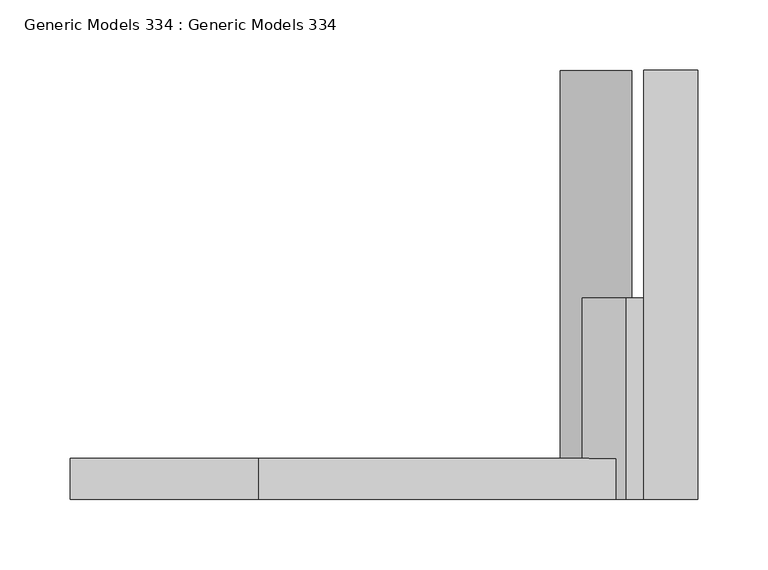
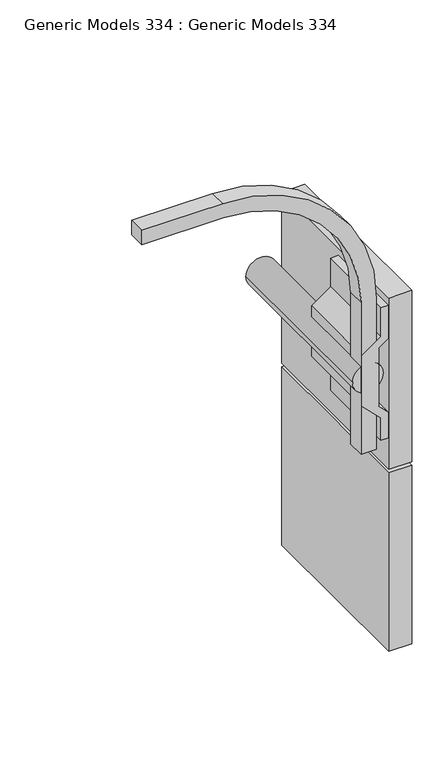
"""IFC4 building model written with IfcOpenShell, lengths in millimetres: proxy geometry, Generic Models 334 : Generic Models 334."""

from ifc_helpers import new_model, si_unit, point, frame, frame_2d, origin, place, context, project, spatial, polyline, circle_curve, trimmed, segment, composite_curve, outline, extrude, source, transform, mapped, element, save


def generic_models_334_generic_models_334_cd4350b1(model_context):
    return source(origin(), model_context, "Body", "SweptSolid", [
        extrude(outline(polyline([(126118.4886506, 8247.7371996), (126175.6386506, 8247.7371996), (126175.6386506, 8235.0371996), (126125.0998522, 8235.0371996), (126103.2465899, 8203.8275067), (126015.1748762, 8203.8275067), (125983.9651833, 8235.0371996), (125944.7756955, 8235.0371996), (125944.7756955, 8247.7371996), (125989.2256955, 8247.7371996), (126005.1885944, 8231.7743007), (126107.3113085, 8231.7743007), (126118.4886506, 8247.7371996)])), frame((0.0, -4109.6428838, 0.0), z_axis=(0.0, 1.0, 0.0), x_axis=(0.0, 0.0, 1.0)), (0.0, 0.0, 1.0), 143.0193921),
        extrude(outline(composite_curve([segment(trimmed(circle_curve(frame_2d((126060.9854905, 8213.7932071)), 25.4), [point((126060.9854905, 8239.1932071))], [point((126060.9854905, 8188.3932071))], False, "CARTESIAN"), True, "CONTINUOUS"), segment(trimmed(circle_curve(frame_2d((126060.9854905, 8213.7932071)), 25.4), [point((126060.9854905, 8188.3932071))], [point((126060.9854905, 8239.1932071))], False, "CARTESIAN"), True, "CONTINUOUS")], self_intersect=False)), frame((0.0, -4109.6428838, 0.0), z_axis=(0.0, 1.0, 0.0), x_axis=(0.0, 0.0, 1.0)), (0.0, 0.0, 1.0), 304.8),
        extrude(outline(composite_curve([segment(trimmed(circle_curve(frame_2d((126194.6886506, 7973.9169406)), 254.0), [point((126194.6886506, 8227.9169406))], [point((126448.6886506, 7973.9169406))], False, "CARTESIAN"), True, "CONTINUOUS"), segment(polyline([(126448.6886506, 7973.9169406), (126448.6886506, 7840.5669406), (126423.2886506, 7840.5669406), (126423.2886506, 7975.117678)]), True, "CONTINUOUS"), segment(trimmed(circle_curve(frame_2d((126194.6886506, 7973.9169406)), 228.6031535), [point((126423.2886506, 7975.117678))], [point((126195.8893881, 8202.5169406))], True, "CARTESIAN"), True, "CONTINUOUS"), segment(polyline([(126195.8893881, 8202.5169406), (125931.2571139, 8202.5169406), (125931.2571139, 8227.9169406), (126194.6886506, 8227.9169406)]), True, "CONTINUOUS")], self_intersect=False)), frame((0.0, -4109.6428838, 0.0), z_axis=(0.0, 1.0, 0.0), x_axis=(0.0, 0.0, 1.0)), (0.0, 0.0, 1.0), 28.9445755),
        extrude(outline(polyline([(8247.7371996, -3804.8428838), (8285.8371996, -3804.8428838), (8285.8371996, -4109.6428838), (8247.7371996, -4109.6428838), (8247.7371996, -3804.8428838)])), frame((0.0, 0.0, 125572.0903036), z_axis=(0.0, 0.0, 1.0), x_axis=(1.0, 0.0, 0.0)), (0.0, 0.0, 1.0), 311.15),
        extrude(outline(polyline([(8247.7371996, -3804.8428838), (8285.8371996, -3804.8428838), (8285.8371996, -4109.6428838), (8247.7371996, -4109.6428838), (8247.7371996, -3804.8428838)])), frame((0.0, 0.0, 125889.5903036), z_axis=(0.0, 0.0, 1.0), x_axis=(1.0, 0.0, 0.0)), (0.0, 0.0, 1.0), 298.45),
    ])


if __name__ == "__main__":
    model = new_model("IFC4")
    model_context = context("Model", 3, world=origin())
    ifc_project = project(units=[si_unit("LENGTHUNIT", "METRE", prefix="MILLI")], contexts=[model_context])
    site = spatial("IfcSite", under=ifc_project)
    building = spatial("IfcBuilding", under=site)
    placement = place(None, origin())
    generic_models_334_generic_models_334_shape = generic_models_334_generic_models_334_cd4350b1(model_context)
    element("IfcBuildingElementProxy", 1, Name="Generic Models 334 : Generic Models 334", ObjectType="Generic Models 334 : Generic Models 334", at=placement, inside=building, context=model_context, shape_type="MappedRepresentation", body=[
        mapped(generic_models_334_generic_models_334_shape, transform((0.0, 0.0, 0.0), x_axis=(1.0, 0.0, 0.0), y_axis=(0.0, 1.0, 0.0), z_axis=(0.0, 0.0, 1.0))),
    ])
    save(model, "model.ifc")

# Revit data of these elements
# Element 1 (IfcBuildingElementProxy, "Generic Models 334 : Generic Models 334")
#   Materials on its faces: "_GARAGE DOOR TRACK", "_SECTIONAL WOODEN GARAGE DOOR PER SCHEDULE"
# Materials
#   "_GARAGE DOOR TRACK": class "Metal", colour RGB 199 199 199, transparency 0, Description = "Structural steel 50ksi", Cost = 0
#   "_SECTIONAL WOODEN GARAGE DOOR PER SCHEDULE": class "Generic", colour RGB 177 130 114, transparency 0, Cost = 0
